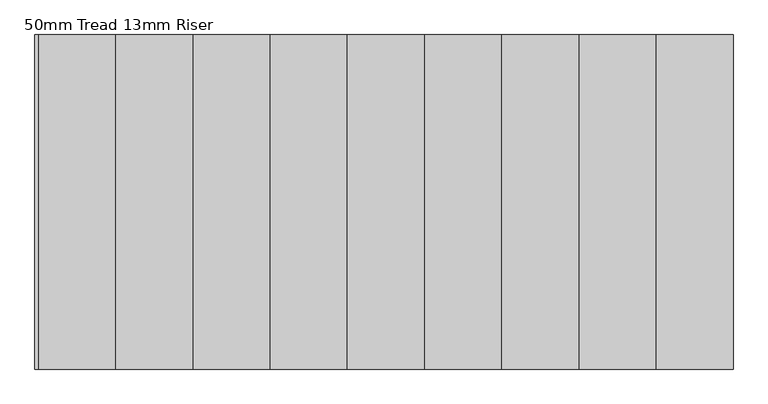
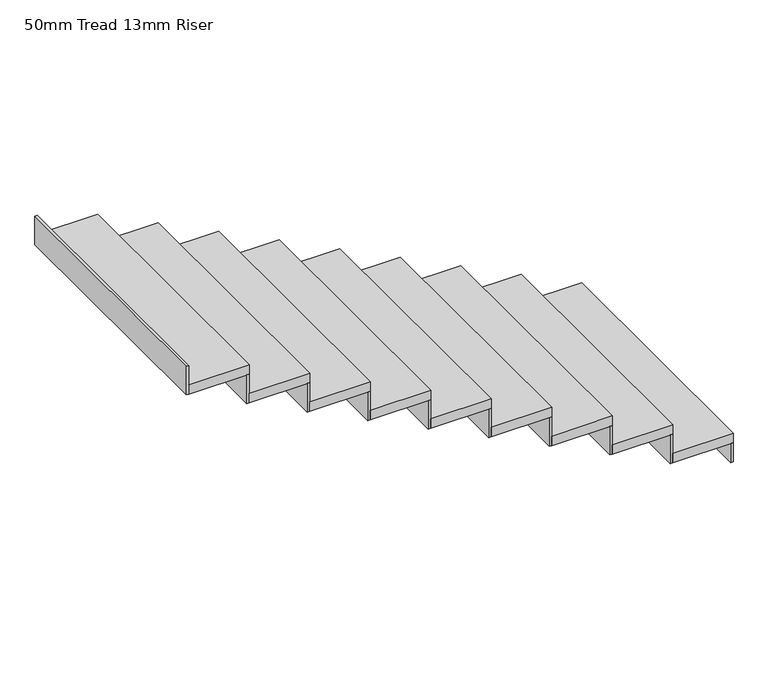
"""IFC4 building model written with IfcOpenShell, lengths in millimetres: stair flight geometry, 50mm Tread 13mm Riser."""

from ifc_helpers import new_model, si_unit, frame, origin, origin_with_axes, place, context, project, spatial, polyline, outline, extrude, source, transform, mapped, element, save


def stair_flight_50mm_tread_13mm_riser_9245e9fd(model_context):
    return source(origin(), model_context, "Body", "SweptSolid", [
        extrude(outline(polyline([(-10508.0859635, -2221.1593564), (-10495.5859635, -2221.1593564), (-10495.5859635, -3521.1593564), (-10508.0859635, -3521.1593564), (-10508.0859635, -2221.1593564)])), origin_with_axes(), (0.0, 0.0, 1.0), 100.0),
        extrude(outline(polyline([(-10795.5859635, -3521.1593564), (-10795.5859635, -2221.1593564), (-10495.5859635, -2221.1593564), (-10495.5859635, -3521.1593564), (-10795.5859635, -3521.1593564)])), frame((0.0, 0.0, 100.0), z_axis=(0.0, 0.0, 1.0), x_axis=(1.0, 0.0, 0.0)), (0.0, 0.0, 1.0), 50.0),
        extrude(outline(polyline([(-10808.0859635, -2221.1593564), (-10795.5859635, -2221.1593564), (-10795.5859635, -3521.1593564), (-10808.0859635, -3521.1593564), (-10808.0859635, -2221.1593564)])), frame((0.0, 0.0, 100.0), z_axis=(0.0, 0.0, 1.0), x_axis=(1.0, 0.0, 0.0)), (0.0, 0.0, 1.0), 150.0),
        extrude(outline(polyline([(-11095.5859635, -3521.1593564), (-11095.5859635, -2221.1593564), (-10795.5859635, -2221.1593564), (-10795.5859635, -3521.1593564), (-11095.5859635, -3521.1593564)])), frame((0.0, 0.0, 250.0), z_axis=(0.0, 0.0, 1.0), x_axis=(1.0, 0.0, 0.0)), (0.0, 0.0, 1.0), 50.0),
        extrude(outline(polyline([(-11108.0859635, -2221.1593564), (-11095.5859635, -2221.1593564), (-11095.5859635, -3521.1593564), (-11108.0859635, -3521.1593564), (-11108.0859635, -2221.1593564)])), frame((0.0, 0.0, 250.0), z_axis=(0.0, 0.0, 1.0), x_axis=(1.0, 0.0, 0.0)), (0.0, 0.0, 1.0), 150.0),
        extrude(outline(polyline([(-11395.5859635, -3521.1593564), (-11395.5859635, -2221.1593564), (-11095.5859635, -2221.1593564), (-11095.5859635, -3521.1593564), (-11395.5859635, -3521.1593564)])), frame((0.0, 0.0, 400.0), z_axis=(0.0, 0.0, 1.0), x_axis=(1.0, 0.0, 0.0)), (0.0, 0.0, 1.0), 50.0),
        extrude(outline(polyline([(-11408.0859635, -2221.1593564), (-11395.5859635, -2221.1593564), (-11395.5859635, -3521.1593564), (-11408.0859635, -3521.1593564), (-11408.0859635, -2221.1593564)])), frame((0.0, 0.0, 400.0), z_axis=(0.0, 0.0, 1.0), x_axis=(1.0, 0.0, 0.0)), (0.0, 0.0, 1.0), 150.0),
        extrude(outline(polyline([(-11695.5859635, -3521.1593564), (-11695.5859635, -2221.1593564), (-11395.5859635, -2221.1593564), (-11395.5859635, -3521.1593564), (-11695.5859635, -3521.1593564)])), frame((0.0, 0.0, 550.0), z_axis=(0.0, 0.0, 1.0), x_axis=(1.0, 0.0, 0.0)), (0.0, 0.0, 1.0), 50.0),
        extrude(outline(polyline([(-11708.0859635, -2221.1593564), (-11695.5859635, -2221.1593564), (-11695.5859635, -3521.1593564), (-11708.0859635, -3521.1593564), (-11708.0859635, -2221.1593564)])), frame((0.0, 0.0, 550.0), z_axis=(0.0, 0.0, 1.0), x_axis=(1.0, 0.0, 0.0)), (0.0, 0.0, 1.0), 150.0),
        extrude(outline(polyline([(-11995.5859635, -3521.1593564), (-11995.5859635, -2221.1593564), (-11695.5859635, -2221.1593564), (-11695.5859635, -3521.1593564), (-11995.5859635, -3521.1593564)])), frame((0.0, 0.0, 700.0), z_axis=(0.0, 0.0, 1.0), x_axis=(1.0, 0.0, 0.0)), (0.0, 0.0, 1.0), 50.0),
        extrude(outline(polyline([(-12008.0859635, -2221.1593564), (-11995.5859635, -2221.1593564), (-11995.5859635, -3521.1593564), (-12008.0859635, -3521.1593564), (-12008.0859635, -2221.1593564)])), frame((0.0, 0.0, 700.0), z_axis=(0.0, 0.0, 1.0), x_axis=(1.0, 0.0, 0.0)), (0.0, 0.0, 1.0), 150.0),
        extrude(outline(polyline([(-12295.5859635, -3521.1593564), (-12295.5859635, -2221.1593564), (-11995.5859635, -2221.1593564), (-11995.5859635, -3521.1593564), (-12295.5859635, -3521.1593564)])), frame((0.0, 0.0, 850.0), z_axis=(0.0, 0.0, 1.0), x_axis=(1.0, 0.0, 0.0)), (0.0, 0.0, 1.0), 50.0),
        extrude(outline(polyline([(-12308.0859635, -2221.1593564), (-12295.5859635, -2221.1593564), (-12295.5859635, -3521.1593564), (-12308.0859635, -3521.1593564), (-12308.0859635, -2221.1593564)])), frame((0.0, 0.0, 850.0), z_axis=(0.0, 0.0, 1.0), x_axis=(1.0, 0.0, 0.0)), (0.0, 0.0, 1.0), 150.0),
        extrude(outline(polyline([(-12595.5859635, -3521.1593564), (-12595.5859635, -2221.1593564), (-12295.5859635, -2221.1593564), (-12295.5859635, -3521.1593564), (-12595.5859635, -3521.1593564)])), frame((0.0, 0.0, 1000.0), z_axis=(0.0, 0.0, 1.0), x_axis=(1.0, 0.0, 0.0)), (0.0, 0.0, 1.0), 50.0),
        extrude(outline(polyline([(-12608.0859635, -2221.1593564), (-12595.5859635, -2221.1593564), (-12595.5859635, -3521.1593564), (-12608.0859635, -3521.1593564), (-12608.0859635, -2221.1593564)])), frame((0.0, 0.0, 1000.0), z_axis=(0.0, 0.0, 1.0), x_axis=(1.0, 0.0, 0.0)), (0.0, 0.0, 1.0), 150.0),
        extrude(outline(polyline([(-12895.5859635, -3521.1593564), (-12895.5859635, -2221.1593564), (-12595.5859635, -2221.1593564), (-12595.5859635, -3521.1593564), (-12895.5859635, -3521.1593564)])), frame((0.0, 0.0, 1150.0), z_axis=(0.0, 0.0, 1.0), x_axis=(1.0, 0.0, 0.0)), (0.0, 0.0, 1.0), 50.0),
        extrude(outline(polyline([(-12908.0859635, -2221.1593564), (-12895.5859635, -2221.1593564), (-12895.5859635, -3521.1593564), (-12908.0859635, -3521.1593564), (-12908.0859635, -2221.1593564)])), frame((0.0, 0.0, 1150.0), z_axis=(0.0, 0.0, 1.0), x_axis=(1.0, 0.0, 0.0)), (0.0, 0.0, 1.0), 150.0),
        extrude(outline(polyline([(-13208.0859635, -2221.1593564), (-13195.5859635, -2221.1593564), (-13195.5859635, -3521.1593564), (-13208.0859635, -3521.1593564), (-13208.0859635, -2221.1593564)])), frame((0.0, 0.0, 1300.0), z_axis=(0.0, 0.0, 1.0), x_axis=(1.0, 0.0, 0.0)), (0.0, 0.0, 1.0), 150.0),
        extrude(outline(polyline([(-13195.5859635, -3521.1593564), (-13195.5859635, -2221.1593564), (-12895.5859635, -2221.1593564), (-12895.5859635, -3521.1593564), (-13195.5859635, -3521.1593564)])), frame((0.0, 0.0, 1300.0), z_axis=(0.0, 0.0, 1.0), x_axis=(1.0, 0.0, 0.0)), (0.0, 0.0, 1.0), 50.0),
    ])


if __name__ == "__main__":
    model = new_model("IFC4")
    model_context = context("Model", 3, world=origin())
    ifc_project = project(units=[si_unit("LENGTHUNIT", "METRE", prefix="MILLI")], contexts=[model_context])
    site = spatial("IfcSite", under=ifc_project)
    building = spatial("IfcBuilding", under=site)
    placement = place(None, origin())
    stair_flight_50mm_tread_13mm_riser_shape = stair_flight_50mm_tread_13mm_riser_9245e9fd(model_context)
    element("IfcStairFlight", 1, ObjectType="50mm Tread 13mm Riser", at=placement, inside=building, context=model_context, shape_type="MappedRepresentation", body=[
        mapped(stair_flight_50mm_tread_13mm_riser_shape, transform((0.0, 0.0, 0.0), x_axis=(1.0, 0.0, 0.0), y_axis=(0.0, 1.0, 0.0), z_axis=(0.0, 0.0, 1.0))),
    ])
    save(model, "model.ifc")
